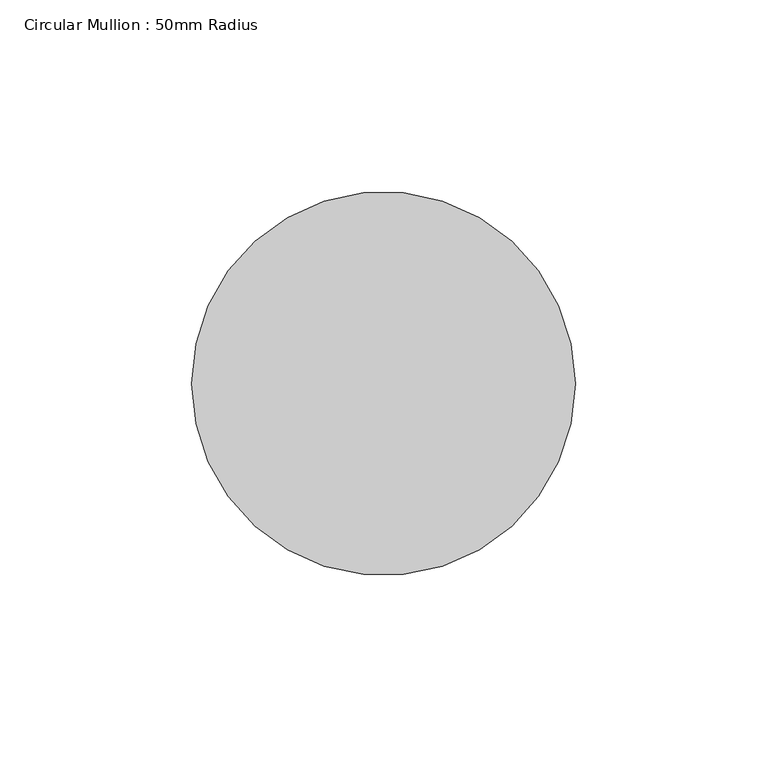
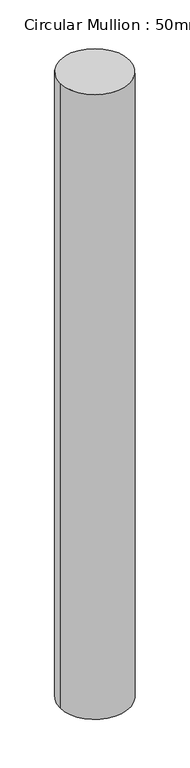
"""IFC4 building model written with IfcOpenShell, lengths in millimetres: member geometry, Circular Mullion : 50mm Radius."""

from ifc_helpers import new_model, si_unit, point, frame, origin, origin_2d, place, context, project, spatial, circle_curve, trimmed, segment, composite_curve, outline, extrude, source, transform, mapped, element, save


def circular_mullion_50mm_radius_9917e02e(model_context):
    return source(origin(), model_context, "Body", "SweptSolid", [
        extrude(outline(composite_curve([segment(trimmed(circle_curve(origin_2d(), 50.0), [point((50.0, 0.0))], [point((-50.0, 0.0))], False, "CARTESIAN"), True, "CONTINUOUS"), segment(trimmed(circle_curve(origin_2d(), 50.0), [point((-50.0, 0.0))], [point((50.0, 0.0))], False, "CARTESIAN"), True, "CONTINUOUS")], self_intersect=False)), frame((0.0, 0.0, -949.4725592), z_axis=(0.0, 0.0, 1.0), x_axis=(1.0, 0.0, 0.0)), (0.0, 0.0, 1.0), 949.4725592),
    ])


if __name__ == "__main__":
    model = new_model("IFC4")
    model_context = context("Model", 3, world=origin())
    ifc_project = project(units=[si_unit("LENGTHUNIT", "METRE", prefix="MILLI")], contexts=[model_context])
    site = spatial("IfcSite", under=ifc_project)
    building = spatial("IfcBuilding", under=site)
    placement = place(None, origin())
    circular_mullion_50mm_radius_shape = circular_mullion_50mm_radius_9917e02e(model_context)
    element("IfcMember", 1, ObjectType="Circular Mullion : 50mm Radius", at=placement, inside=building, context=model_context, shape_type="MappedRepresentation", body=[
        mapped(circular_mullion_50mm_radius_shape, transform((0.0, 0.0, 0.0), x_axis=(1.0, 0.0, 0.0), y_axis=(0.0, 1.0, 0.0), z_axis=(0.0, 0.0, 1.0))),
    ])
    save(model, "model.ifc")

# Revit data of these elements
# Type "Circular Mullion : 50mm Radius"
#   built-in parameter 1007350 = 0.164042 (stored number, unit not read)
# Element 1 (IfcMember, "Circular Mullion : 50mm Radius")
#   Materials on its faces: "Aluminium"
# Materials
#   "Aluminium": class "Metal", colour RGB 247 247 247, transparency 0, Description = "Aluminium 6061", Cost = 0
